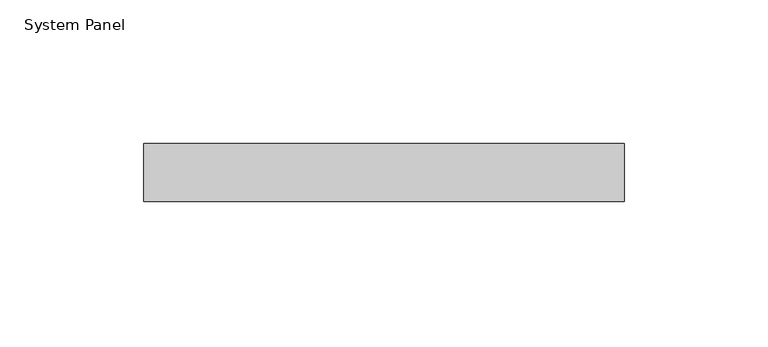
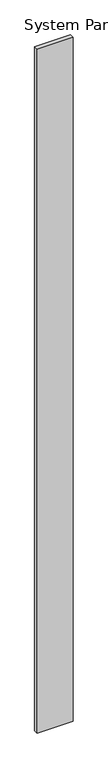
"""IFC4 building model written with IfcOpenShell, lengths in millimetres: plate geometry, System Panel : WWm-Glass-20mm-10mmOffset."""

import ifcopenshell
import ifcopenshell.guid

model = None  # the IFC model being written
_history = None  # IfcOwnerHistory: only IFC2X3 demands one
_inside = {}  # id of a spatial element -> (the spatial element, [elements in it])
_under = {}  # id of a project, library or spatial element -> (it, [spatial elements below it])
_declared = {}  # id of a project -> (the project, [libraries it declares])
_typed = {}  # id of a type object -> (the type object, [elements of that type])
_made_of = {}  # id of a material, layer set ... -> (it, [elements and type objects made of it])


def new_model(schema):
    """Start an empty IFC model of exactly this schema.

    Asked for "IFC4X3", IfcOpenShell would pick the latest addendum, in which some entities
    have other attributes; the version numbers below select the first issue.
    IFC2X3 requires an IfcOwnerHistory on every rooted entity: one is made here for all.
    """
    global model, _history
    if schema == "IFC4X3":
        model = ifcopenshell.file(schema_version=(4, 3, 0, 0))
    else:
        model = ifcopenshell.file(schema=schema)
    _inside.clear()
    _under.clear()
    _declared.clear()
    _typed.clear()
    _made_of.clear()
    _history = None
    if model.schema == "IFC2X3":
        org = make("IfcOrganization", Name="unknown")
        user = make(
            "IfcPersonAndOrganization",
            ThePerson=make("IfcPerson", FamilyName="unknown"),
            TheOrganization=org,
        )
        app = make(
            "IfcApplication",
            ApplicationDeveloper=org,
            Version="unknown",
            ApplicationFullName="unknown",
            ApplicationIdentifier="unknown",
        )
        _history = make(
            "IfcOwnerHistory",
            OwningUser=user,
            OwningApplication=app,
            ChangeAction="ADDED",
            CreationDate=0,
        )
    return model


def make(cls, **values):
    """One entity of the class cls with the attributes given. An attribute that is None is left unset."""
    return model.create_entity(
        cls, **{name: value for name, value in values.items() if value is not None}
    )


def rooted(cls, **values):
    """An entity with a GlobalId (a new one), such as an element, a storey or a relation."""
    return make(cls, GlobalId=ifcopenshell.guid.new(), OwnerHistory=_history, **values)


def si_unit(unit_type, name, prefix=None):
    """IfcSIUnit, for example si_unit("LENGTHUNIT", "METRE", prefix="MILLI")."""
    return make("IfcSIUnit", UnitType=unit_type, Prefix=prefix, Name=name)


def assignment(units):
    """IfcUnitAssignment: the units of a project."""
    return None if units is None else make("IfcUnitAssignment", Units=units)


def point(xyz):
    """IfcCartesianPoint."""
    return None if xyz is None else make("IfcCartesianPoint", Coordinates=xyz)


def direction(xyz):
    """IfcDirection."""
    return None if xyz is None else make("IfcDirection", DirectionRatios=xyz)


def frame(location, z_axis=None, x_axis=None):
    """IfcAxis2Placement3D, a coordinate frame: its origin and axes. An axis left out is left unset."""
    return make(
        "IfcAxis2Placement3D",
        Location=point(location),
        Axis=direction(z_axis),
        RefDirection=direction(x_axis),
    )


def origin():
    """The frame at (0, 0, 0) with its axes left unset."""
    return frame((0.0, 0.0, 0.0))


def origin_with_axes():
    """The frame at (0, 0, 0) with the z axis (0, 0, 1) and the x axis (1, 0, 0) written out."""
    return frame((0.0, 0.0, 0.0), z_axis=(0.0, 0.0, 1.0), x_axis=(1.0, 0.0, 0.0))


def place(relative_to, where):
    """IfcLocalPlacement: puts the frame where relative to a parent placement (None: the world)."""
    return make(
        "IfcLocalPlacement", PlacementRelTo=relative_to, RelativePlacement=where
    )


def context(
    kind, dimensions, precision=None, world=None, true_north=None, identifier=None
):
    """IfcGeometricRepresentationContext, for example the 3D "Model" context."""
    return make(
        "IfcGeometricRepresentationContext",
        ContextIdentifier=identifier,
        ContextType=kind,
        CoordinateSpaceDimension=dimensions,
        Precision=precision,
        WorldCoordinateSystem=world,
        TrueNorth=true_north,
    )


def project(units=None, contexts=None):
    """IfcProject with its units and contexts."""
    return rooted(
        "IfcProject",
        Name="project",
        RepresentationContexts=contexts,
        UnitsInContext=assignment(units),
    )


def spatial(cls, under=None, at=None, **own):
    """A site, building, storey or space (cls), placed at a placement, below another one or the project."""
    s = rooted(cls, ObjectPlacement=at, **own)
    if under is not None:
        _under.setdefault(under.id(), (under, []))[1].append(s)
    return s


def polyline(points):
    """IfcPolyline through the points."""
    return make("IfcPolyline", Points=[point(p) for p in points])


def outline(outer, holes=None, kind="AREA"):
    """IfcArbitraryClosedProfileDef: a profile drawn as a closed curve; with holes, ...WithVoids."""
    if holes is None:
        return make("IfcArbitraryClosedProfileDef", ProfileType=kind, OuterCurve=outer)
    return make(
        "IfcArbitraryProfileDefWithVoids",
        ProfileType=kind,
        OuterCurve=outer,
        InnerCurves=holes,
    )


def extrude(swept, where, along, depth):
    """IfcExtrudedAreaSolid: the profile swept, set in the frame where, extruded along a direction by depth."""
    return make(
        "IfcExtrudedAreaSolid",
        SweptArea=swept,
        Position=where,
        ExtrudedDirection=direction(along),
        Depth=depth,
    )


def shape(context_of_items, identifier, shape_type, items):
    """IfcShapeRepresentation: the items that make up one representation, for example the "Body"."""
    return make(
        "IfcShapeRepresentation",
        ContextOfItems=context_of_items,
        RepresentationIdentifier=identifier,
        RepresentationType=shape_type,
        Items=items,
    )


def source(mapping_origin, context_of_items, identifier, shape_type, items):
    """IfcRepresentationMap: a shape defined once, which mapped items show again and again."""
    return make(
        "IfcRepresentationMap",
        MappingOrigin=mapping_origin,
        MappedRepresentation=shape(context_of_items, identifier, shape_type, items),
    )


def transform(
    local_origin,
    x_axis=None,
    y_axis=None,
    z_axis=None,
    scale=None,
    scale2=None,
    scale3=None,
    uniform=True,
):
    """IfcCartesianTransformationOperator3D, or its non-uniform kind. x_axis, y_axis, z_axis: its Axis1, 2, 3."""
    if uniform:
        return make(
            "IfcCartesianTransformationOperator3D",
            Axis1=direction(x_axis),
            Axis2=direction(y_axis),
            LocalOrigin=point(local_origin),
            Scale=scale,
            Axis3=direction(z_axis),
        )
    return make(
        "IfcCartesianTransformationOperator3DnonUniform",
        Axis1=direction(x_axis),
        Axis2=direction(y_axis),
        LocalOrigin=point(local_origin),
        Scale=scale,
        Axis3=direction(z_axis),
        Scale2=scale2,
        Scale3=scale3,
    )


def mapped(mapping_source, mapping_target):
    """IfcMappedItem: shows the shape of a source again, moved by a transform."""
    return make(
        "IfcMappedItem", MappingSource=mapping_source, MappingTarget=mapping_target
    )


def made_of(thing, what):
    """Note that an element or type object is made of a material, layer set ...; save() writes the relation."""
    if what is not None:
        _made_of.setdefault(what.id(), (what, []))[1].append(thing)
    return thing


def element(
    cls,
    number,
    at=None,
    inside=None,
    cuts=None,
    type_object=None,
    material=None,
    context=None,
    identifier="Body",
    shape_type=None,
    held_by="IfcProductDefinitionShape",
    body=None,
    shapes=None,
    **own,
):
    """One element of the class cls, such as IfcWall. Its Tag is "e" and its number.

    at: its placement. inside: the storey or other place that contains it. cuts: it is an
    opening in that element (IfcRelVoidsElement). A single representation is given by context,
    identifier, shape_type and body (its items); several are given by shapes. held_by: the class
    of the entity that holds the representations. save() writes the other relations.
    """
    e = rooted(cls, Tag="e%d" % number, ObjectPlacement=at, **own)
    if body is not None:
        shapes = [shape(context, identifier, shape_type, body)]
    if shapes is not None:
        e.Representation = make(held_by, Representations=shapes)
    if inside is not None:
        _inside.setdefault(inside.id(), (inside, []))[1].append(e)
    if cuts is not None:
        rooted(
            "IfcRelVoidsElement", RelatingBuildingElement=cuts, RelatedOpeningElement=e
        )
    if type_object is not None:
        _typed.setdefault(type_object.id(), (type_object, []))[1].append(e)
    return made_of(e, material)


def aggregate(whole, parts):
    """IfcRelAggregates: a whole, such as a stair, and the parts it consists of."""
    return rooted("IfcRelAggregates", RelatingObject=whole, RelatedObjects=parts)


def save(model, path):
    """Write the relations noted so far, then the file.

    IfcRelAggregates (storeys below a building ...), IfcRelContainedInSpatialStructure (elements
    in a storey), IfcRelDefinesByType, IfcRelAssociatesMaterial and IfcRelDeclares: one each for
    every whole, place, type object, material and project.
    """
    for whole, parts in _under.values():
        aggregate(whole, parts)
    for where, things in _inside.values():
        rooted(
            "IfcRelContainedInSpatialStructure",
            RelatedElements=things,
            RelatingStructure=where,
        )
    for kind, things in _typed.values():
        rooted("IfcRelDefinesByType", RelatedObjects=things, RelatingType=kind)
    for what, things in _made_of.values():
        rooted("IfcRelAssociatesMaterial", RelatedObjects=things, RelatingMaterial=what)
    for by, libraries in _declared.values():
        rooted("IfcRelDeclares", RelatingContext=by, RelatedDefinitions=libraries)
    model.write(path)


def system_panel_9f61c7e3(model_context):
    return source(origin(), model_context, "Body", "SweptSolid", [
        extrude(outline(polyline([(83.385636, 0.0), (-83.385636, 0.0), (-83.385636, 20.0), (83.385636, 20.0), (83.385636, 0.0)])), origin_with_axes(), (0.0, 0.0, 1.0), 3350.0),
    ])


if __name__ == "__main__":
    model = new_model("IFC4")
    model_context = context("Model", 3, world=origin())
    ifc_project = project(units=[si_unit("LENGTHUNIT", "METRE", prefix="MILLI")], contexts=[model_context])
    site = spatial("IfcSite", under=ifc_project)
    building = spatial("IfcBuilding", under=site)
    placement = place(None, origin())
    system_panel_shape = system_panel_9f61c7e3(model_context)
    element("IfcPlate", 1, ObjectType="System Panel : WWm-Glass-20mm-10mmOffset", at=placement, inside=building, context=model_context, shape_type="MappedRepresentation", body=[
        mapped(system_panel_shape, transform((0.0, 0.0, 0.0), x_axis=(1.0, 0.0, 0.0), y_axis=(0.0, 1.0, 0.0), z_axis=(0.0, 0.0, 1.0))),
    ])
    save(model, "model.ifc")

# Revit data of these elements
# Type "System Panel : WWm-Glass-20mm-10mmOffset"
#   Finish = ""
# Element 1 (IfcPlate, "System Panel : WWm-Glass-20mm-10mmOffset")
#   Materials on its faces: "WW-EC-GL-Storefront"
# Materials
#   "WW-EC-GL-Storefront": class "Glass", colour RGB 236 240 239, transparency 0.85, Description = "Storefront Glass", Cost = 0
